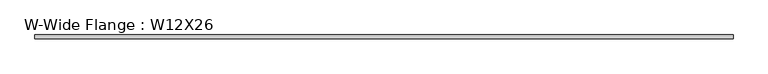
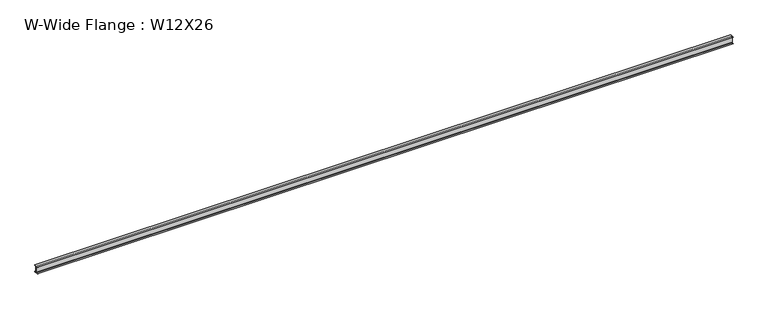
"""IFC4 building model written with IfcOpenShell, lengths in millimetres: beam geometry, W-Wide Flange : W12X26."""

from ifc_helpers import new_model, si_unit, point, frame, frame_2d, origin, place, context, project, spatial, polyline, circle_curve, trimmed, segment, composite_curve, outline, extrude, source, transform, mapped, element, save


def w_wide_flange_w12x26_f353fd54(model_context):
    return source(origin(), model_context, "Body", "SweptSolid", [
        extrude(outline(composite_curve([segment(polyline([(82.4011719, -145.5539063), (82.4011719, -155.178125), (-82.4011719, -155.178125), (-82.4011719, -145.5539063), (-20.2902344, -145.5539063)]), True, "CONTINUOUS"), segment(trimmed(circle_curve(frame_2d((-20.2902344, -128.190625)), 17.3632812), [point((-20.2902344, -145.5539063))], [point((-2.9269531, -128.190625))], True, "CARTESIAN"), True, "CONTINUOUS"), segment(polyline([(-2.9269531, -128.190625), (-2.9269531, 128.190625)]), True, "CONTINUOUS"), segment(trimmed(circle_curve(frame_2d((-20.2902344, 128.190625)), 17.3632812), [point((-2.9269531, 128.190625))], [point((-20.2902344, 145.5539062))], True, "CARTESIAN"), True, "CONTINUOUS"), segment(polyline([(-20.2902344, 145.5539062), (-82.4011719, 145.5539062), (-82.4011719, 155.178125), (82.4011719, 155.178125), (82.4011719, 145.5539062), (20.2902344, 145.5539062)]), True, "CONTINUOUS"), segment(trimmed(circle_curve(frame_2d((20.2902344, 128.190625)), 17.3632812), [point((20.2902344, 145.5539062))], [point((2.9269531, 128.190625))], True, "CARTESIAN"), True, "CONTINUOUS"), segment(polyline([(2.9269531, 128.190625), (2.9269531, -128.190625)]), True, "CONTINUOUS"), segment(trimmed(circle_curve(frame_2d((20.2902344, -128.190625)), 17.3632812), [point((2.9269531, -128.190625))], [point((20.2902344, -145.5539063))], True, "CARTESIAN"), True, "CONTINUOUS"), segment(polyline([(20.2902344, -145.5539063), (82.4011719, -145.5539063)]), True, "CONTINUOUS")], self_intersect=False)), frame((-15240.0, 0.0, 0.0), z_axis=(1.0, 0.0, 0.0), x_axis=(0.0, 1.0, 0.0)), (0.0, 0.0, 1.0), 30480.0),
    ])


if __name__ == "__main__":
    model = new_model("IFC4")
    model_context = context("Model", 3, world=origin())
    ifc_project = project(units=[si_unit("LENGTHUNIT", "METRE", prefix="MILLI")], contexts=[model_context])
    site = spatial("IfcSite", under=ifc_project)
    building = spatial("IfcBuilding", under=site)
    placement = place(None, origin())
    w_wide_flange_w12x26_shape = w_wide_flange_w12x26_f353fd54(model_context)
    element("IfcBeam", 1, ObjectType="W-Wide Flange : W12X26", at=placement, inside=building, context=model_context, shape_type="MappedRepresentation", body=[
        mapped(w_wide_flange_w12x26_shape, transform((0.0, 0.0, 0.0), x_axis=(1.0, 0.0, 0.0), y_axis=(0.0, 1.0, 0.0), z_axis=(0.0, 0.0, 1.0))),
    ])
    save(model, "model.ifc")

# Revit data of these elements
# Type "W-Wide Flange : W12X26"
#   Assembly Code = "B10"
#   W = 26
#   Length [instance default] = 5' - 0"
#   bf = 0' - 6 125/256"
#   d = 1' - 0 7/32"
#   k = 0' - 1 1/16"
#   k2 = 0' - 0 175/256"
#   tf = 0' - 0 97/256"
#   tw = 0' - 0 59/256"
#   A = 0.053125 SF
#   Structural Material [instance default] = none
